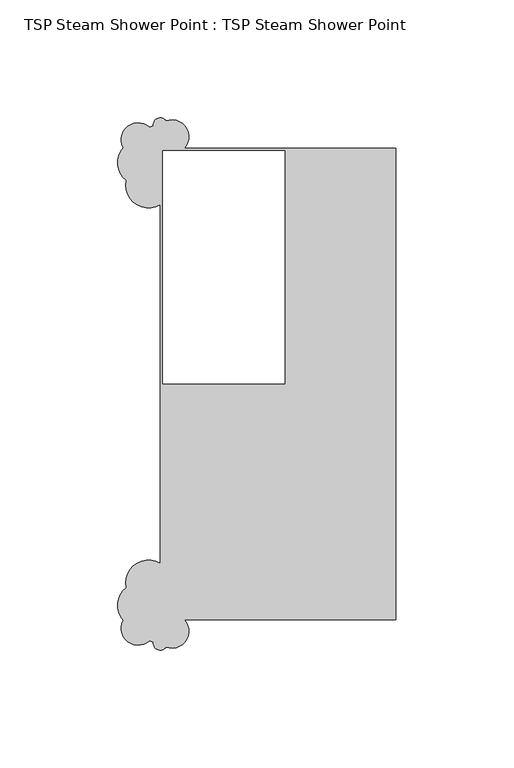
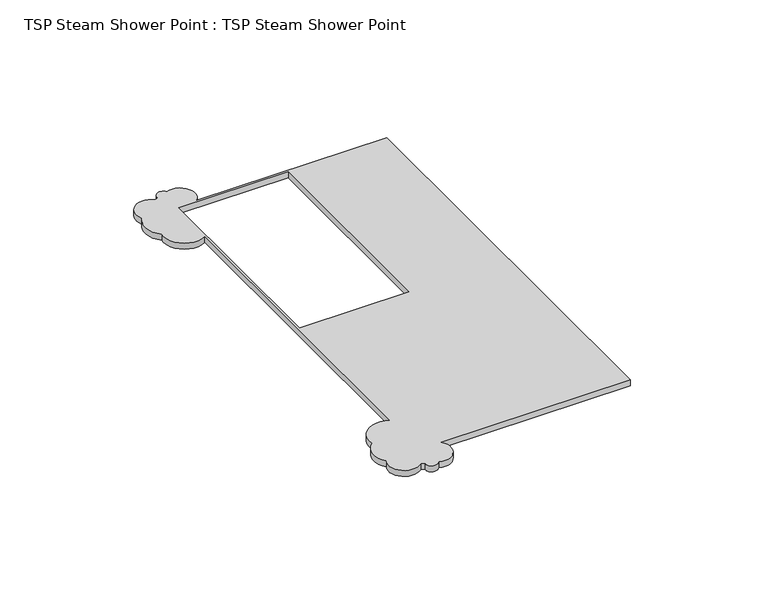
"""IFC4 building model written with IfcOpenShell, lengths in millimetres: proxy geometry, TSP Steam Shower Point : TSP Steam Shower Point."""

from ifc_helpers import new_model, si_unit, point, frame_2d, origin, origin_with_axes, place, context, project, spatial, polyline, circle_curve, trimmed, segment, composite_curve, outline, extrude, source, transform, mapped, element, save


def tsp_steam_shower_point_tsp_steam_shower_point_fb01362a(model_context):
    return source(origin(), model_context, "Body", "SweptSolid", [
        extrude(outline(composite_curve([segment(polyline([(-89.8606046, 100.0), (0.0, 100.0), (0.0, -100.0), (-89.8606046, -100.0)]), True, "CONTINUOUS"), segment(trimmed(circle_curve(frame_2d((-95.0181747, -104.9418108)), 7.1429702), [point((-89.8606046, -100.0))], [point((-97.5633366, -111.6159529))], False, "CARTESIAN"), True, "CONTINUOUS"), segment(trimmed(circle_curve(frame_2d((-100.0, -110.0)), 2.9238044), [point((-97.5633366, -111.6159529))], [point((-102.8923925, -109.5725684))], False, "CARTESIAN"), True, "CONTINUOUS"), segment(trimmed(circle_curve(frame_2d((-100.0, -100.0)), 10.0), [point((-102.8923925, -109.5725684))], [point((-104.4956441, -108.9324792))], False, "CARTESIAN"), True, "CONTINUOUS"), segment(trimmed(circle_curve(frame_2d((-109.329865, -103.5991137)), 7.1982275), [point((-104.4956441, -108.9324792))], [point((-115.7422421, -100.3286554))], False, "CARTESIAN"), True, "CONTINUOUS"), segment(trimmed(circle_curve(frame_2d((-107.9998205, -93.9997607)), 10.0), [point((-115.7422421, -100.3286554))], [point((-114.4638454, -86.3697946))], False, "CARTESIAN"), True, "CONTINUOUS"), segment(trimmed(circle_curve(frame_2d((-104.8816287, -84.4983461)), 9.7632574), [point((-114.4638454, -86.3697946))], [point((-100.0, -76.0431171))], False, "CARTESIAN"), True, "CONTINUOUS"), segment(polyline([(-100.0, -76.0431171), (-100.0, 76.0431171)]), True, "CONTINUOUS"), segment(trimmed(circle_curve(frame_2d((-104.8816287, 84.4983461)), 9.7632574), [point((-100.0, 76.0431171))], [point((-114.4638454, 86.3697946))], False, "CARTESIAN"), True, "CONTINUOUS"), segment(trimmed(circle_curve(frame_2d((-107.9998205, 93.9997607)), 10.0), [point((-114.4638454, 86.3697946))], [point((-115.7422421, 100.3286554))], False, "CARTESIAN"), True, "CONTINUOUS"), segment(trimmed(circle_curve(frame_2d((-109.329865, 103.5991137)), 7.1982275), [point((-115.7422421, 100.3286554))], [point((-104.4956441, 108.9324792))], False, "CARTESIAN"), True, "CONTINUOUS"), segment(trimmed(circle_curve(frame_2d((-100.0, 100.0)), 10.0), [point((-104.4956441, 108.9324792))], [point((-102.8923925, 109.5725684))], False, "CARTESIAN"), True, "CONTINUOUS"), segment(trimmed(circle_curve(frame_2d((-100.0, 110.0)), 2.9238044), [point((-102.8923925, 109.5725684))], [point((-97.5633366, 111.6159529))], False, "CARTESIAN"), True, "CONTINUOUS"), segment(trimmed(circle_curve(frame_2d((-95.0181747, 104.9418108)), 7.1429702), [point((-97.5633366, 111.6159529))], [point((-89.8606046, 100.0))], False, "CARTESIAN"), True, "CONTINUOUS")], self_intersect=False), holes=[polyline([(-99.0, 0.0), (-47.2426407, 0.0), (-47.2426407, 99.0), (-99.0, 99.0), (-99.0, 0.0)])]), origin_with_axes(), (0.0, 0.0, 1.0), 3.0),
    ])


if __name__ == "__main__":
    model = new_model("IFC4")
    model_context = context("Model", 3, world=origin())
    ifc_project = project(units=[si_unit("LENGTHUNIT", "METRE", prefix="MILLI")], contexts=[model_context])
    site = spatial("IfcSite", under=ifc_project)
    building = spatial("IfcBuilding", under=site)
    placement = place(None, origin())
    tsp_steam_shower_point_tsp_steam_shower_point_shape = tsp_steam_shower_point_tsp_steam_shower_point_fb01362a(model_context)
    element("IfcBuildingElementProxy", 1, Name="TSP Steam Shower Point : TSP Steam Shower Point", ObjectType="TSP Steam Shower Point : TSP Steam Shower Point", at=placement, inside=building, context=model_context, shape_type="MappedRepresentation", body=[
        mapped(tsp_steam_shower_point_tsp_steam_shower_point_shape, transform((0.0, 0.0, 0.0), x_axis=(1.0, 0.0, 0.0), y_axis=(0.0, 1.0, 0.0), z_axis=(0.0, 0.0, 1.0))),
    ])
    save(model, "model.ifc")

# Revit data of these elements
# Type "TSP Steam Shower Point : TSP Steam Shower Point"
#   Model = "TSP_ELECSSHR"
#   Default Elevation = 0
# Element 1 (IfcBuildingElementProxy, "TSP Steam Shower Point : TSP Steam Shower Point")
#   Materials on its faces: "Plastic, Opaque Black"
# Materials
#   "Plastic, Opaque Black": class "Plastic", colour RGB 0 0 0, transparency 0.7, Description = "Plastic, generic, opaque black", Cost = 0
